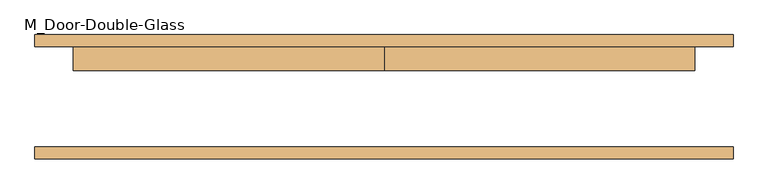
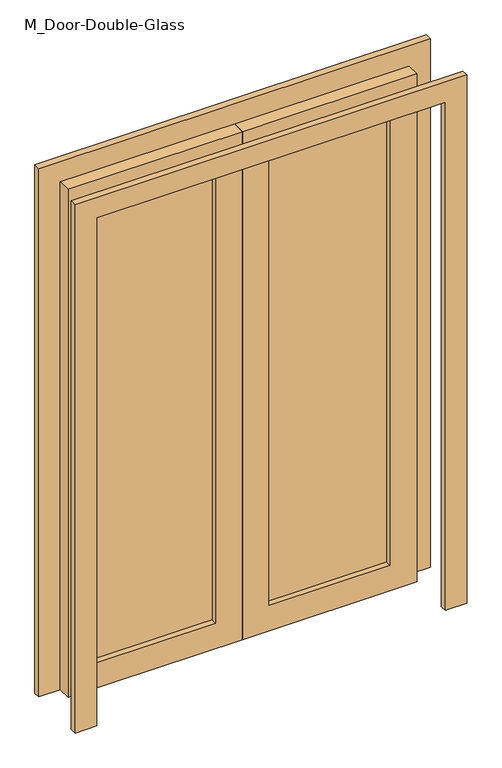
"""IFC4 building model written with IfcOpenShell, lengths in millimetres: door geometry, M_Door-Double-Glass : 130x210cm Kapı."""

import ifcopenshell
import ifcopenshell.guid

model = None  # the IFC model being written
_history = None  # IfcOwnerHistory: only IFC2X3 demands one
_inside = {}  # id of a spatial element -> (the spatial element, [elements in it])
_under = {}  # id of a project, library or spatial element -> (it, [spatial elements below it])
_declared = {}  # id of a project -> (the project, [libraries it declares])
_typed = {}  # id of a type object -> (the type object, [elements of that type])
_made_of = {}  # id of a material, layer set ... -> (it, [elements and type objects made of it])


def new_model(schema):
    """Start an empty IFC model of exactly this schema.

    Asked for "IFC4X3", IfcOpenShell would pick the latest addendum, in which some entities
    have other attributes; the version numbers below select the first issue.
    IFC2X3 requires an IfcOwnerHistory on every rooted entity: one is made here for all.
    """
    global model, _history
    if schema == "IFC4X3":
        model = ifcopenshell.file(schema_version=(4, 3, 0, 0))
    else:
        model = ifcopenshell.file(schema=schema)
    _inside.clear()
    _under.clear()
    _declared.clear()
    _typed.clear()
    _made_of.clear()
    _history = None
    if model.schema == "IFC2X3":
        org = make("IfcOrganization", Name="unknown")
        user = make(
            "IfcPersonAndOrganization",
            ThePerson=make("IfcPerson", FamilyName="unknown"),
            TheOrganization=org,
        )
        app = make(
            "IfcApplication",
            ApplicationDeveloper=org,
            Version="unknown",
            ApplicationFullName="unknown",
            ApplicationIdentifier="unknown",
        )
        _history = make(
            "IfcOwnerHistory",
            OwningUser=user,
            OwningApplication=app,
            ChangeAction="ADDED",
            CreationDate=0,
        )
    return model


def make(cls, **values):
    """One entity of the class cls with the attributes given. An attribute that is None is left unset."""
    return model.create_entity(
        cls, **{name: value for name, value in values.items() if value is not None}
    )


def rooted(cls, **values):
    """An entity with a GlobalId (a new one), such as an element, a storey or a relation."""
    return make(cls, GlobalId=ifcopenshell.guid.new(), OwnerHistory=_history, **values)


def si_unit(unit_type, name, prefix=None):
    """IfcSIUnit, for example si_unit("LENGTHUNIT", "METRE", prefix="MILLI")."""
    return make("IfcSIUnit", UnitType=unit_type, Prefix=prefix, Name=name)


def assignment(units):
    """IfcUnitAssignment: the units of a project."""
    return None if units is None else make("IfcUnitAssignment", Units=units)


def point(xyz):
    """IfcCartesianPoint."""
    return None if xyz is None else make("IfcCartesianPoint", Coordinates=xyz)


def direction(xyz):
    """IfcDirection."""
    return None if xyz is None else make("IfcDirection", DirectionRatios=xyz)


def frame(location, z_axis=None, x_axis=None):
    """IfcAxis2Placement3D, a coordinate frame: its origin and axes. An axis left out is left unset."""
    return make(
        "IfcAxis2Placement3D",
        Location=point(location),
        Axis=direction(z_axis),
        RefDirection=direction(x_axis),
    )


def origin():
    """The frame at (0, 0, 0) with its axes left unset."""
    return frame((0.0, 0.0, 0.0))


def place(relative_to, where):
    """IfcLocalPlacement: puts the frame where relative to a parent placement (None: the world)."""
    return make(
        "IfcLocalPlacement", PlacementRelTo=relative_to, RelativePlacement=where
    )


def context(
    kind, dimensions, precision=None, world=None, true_north=None, identifier=None
):
    """IfcGeometricRepresentationContext, for example the 3D "Model" context."""
    return make(
        "IfcGeometricRepresentationContext",
        ContextIdentifier=identifier,
        ContextType=kind,
        CoordinateSpaceDimension=dimensions,
        Precision=precision,
        WorldCoordinateSystem=world,
        TrueNorth=true_north,
    )


def project(units=None, contexts=None):
    """IfcProject with its units and contexts."""
    return rooted(
        "IfcProject",
        Name="project",
        RepresentationContexts=contexts,
        UnitsInContext=assignment(units),
    )


def spatial(cls, under=None, at=None, **own):
    """A site, building, storey or space (cls), placed at a placement, below another one or the project."""
    s = rooted(cls, ObjectPlacement=at, **own)
    if under is not None:
        _under.setdefault(under.id(), (under, []))[1].append(s)
    return s


def polyline(points):
    """IfcPolyline through the points."""
    return make("IfcPolyline", Points=[point(p) for p in points])


def outline(outer, holes=None, kind="AREA"):
    """IfcArbitraryClosedProfileDef: a profile drawn as a closed curve; with holes, ...WithVoids."""
    if holes is None:
        return make("IfcArbitraryClosedProfileDef", ProfileType=kind, OuterCurve=outer)
    return make(
        "IfcArbitraryProfileDefWithVoids",
        ProfileType=kind,
        OuterCurve=outer,
        InnerCurves=holes,
    )


def extrude(swept, where, along, depth):
    """IfcExtrudedAreaSolid: the profile swept, set in the frame where, extruded along a direction by depth."""
    return make(
        "IfcExtrudedAreaSolid",
        SweptArea=swept,
        Position=where,
        ExtrudedDirection=direction(along),
        Depth=depth,
    )


def shape(context_of_items, identifier, shape_type, items):
    """IfcShapeRepresentation: the items that make up one representation, for example the "Body"."""
    return make(
        "IfcShapeRepresentation",
        ContextOfItems=context_of_items,
        RepresentationIdentifier=identifier,
        RepresentationType=shape_type,
        Items=items,
    )


def source(mapping_origin, context_of_items, identifier, shape_type, items):
    """IfcRepresentationMap: a shape defined once, which mapped items show again and again."""
    return make(
        "IfcRepresentationMap",
        MappingOrigin=mapping_origin,
        MappedRepresentation=shape(context_of_items, identifier, shape_type, items),
    )


def transform(
    local_origin,
    x_axis=None,
    y_axis=None,
    z_axis=None,
    scale=None,
    scale2=None,
    scale3=None,
    uniform=True,
):
    """IfcCartesianTransformationOperator3D, or its non-uniform kind. x_axis, y_axis, z_axis: its Axis1, 2, 3."""
    if uniform:
        return make(
            "IfcCartesianTransformationOperator3D",
            Axis1=direction(x_axis),
            Axis2=direction(y_axis),
            LocalOrigin=point(local_origin),
            Scale=scale,
            Axis3=direction(z_axis),
        )
    return make(
        "IfcCartesianTransformationOperator3DnonUniform",
        Axis1=direction(x_axis),
        Axis2=direction(y_axis),
        LocalOrigin=point(local_origin),
        Scale=scale,
        Axis3=direction(z_axis),
        Scale2=scale2,
        Scale3=scale3,
    )


def mapped(mapping_source, mapping_target):
    """IfcMappedItem: shows the shape of a source again, moved by a transform."""
    return make(
        "IfcMappedItem", MappingSource=mapping_source, MappingTarget=mapping_target
    )


def made_of(thing, what):
    """Note that an element or type object is made of a material, layer set ...; save() writes the relation."""
    if what is not None:
        _made_of.setdefault(what.id(), (what, []))[1].append(thing)
    return thing


def element(
    cls,
    number,
    at=None,
    inside=None,
    cuts=None,
    type_object=None,
    material=None,
    context=None,
    identifier="Body",
    shape_type=None,
    held_by="IfcProductDefinitionShape",
    body=None,
    shapes=None,
    **own,
):
    """One element of the class cls, such as IfcWall. Its Tag is "e" and its number.

    at: its placement. inside: the storey or other place that contains it. cuts: it is an
    opening in that element (IfcRelVoidsElement). A single representation is given by context,
    identifier, shape_type and body (its items); several are given by shapes. held_by: the class
    of the entity that holds the representations. save() writes the other relations.
    """
    e = rooted(cls, Tag="e%d" % number, ObjectPlacement=at, **own)
    if body is not None:
        shapes = [shape(context, identifier, shape_type, body)]
    if shapes is not None:
        e.Representation = make(held_by, Representations=shapes)
    if inside is not None:
        _inside.setdefault(inside.id(), (inside, []))[1].append(e)
    if cuts is not None:
        rooted(
            "IfcRelVoidsElement", RelatingBuildingElement=cuts, RelatedOpeningElement=e
        )
    if type_object is not None:
        _typed.setdefault(type_object.id(), (type_object, []))[1].append(e)
    return made_of(e, material)


def aggregate(whole, parts):
    """IfcRelAggregates: a whole, such as a stair, and the parts it consists of."""
    return rooted("IfcRelAggregates", RelatingObject=whole, RelatedObjects=parts)


def save(model, path):
    """Write the relations noted so far, then the file.

    IfcRelAggregates (storeys below a building ...), IfcRelContainedInSpatialStructure (elements
    in a storey), IfcRelDefinesByType, IfcRelAssociatesMaterial and IfcRelDeclares: one each for
    every whole, place, type object, material and project.
    """
    for whole, parts in _under.values():
        aggregate(whole, parts)
    for where, things in _inside.values():
        rooted(
            "IfcRelContainedInSpatialStructure",
            RelatedElements=things,
            RelatingStructure=where,
        )
    for kind, things in _typed.values():
        rooted("IfcRelDefinesByType", RelatedObjects=things, RelatingType=kind)
    for what, things in _made_of.values():
        rooted("IfcRelAssociatesMaterial", RelatedObjects=things, RelatingMaterial=what)
    for by, libraries in _declared.values():
        rooted("IfcRelDeclares", RelatingContext=by, RelatedDefinitions=libraries)
    model.write(path)


def m_door_double_glass_87eabaac(model_context):
    return source(origin(), model_context, "Body", "SweptSolid", [
        extrude(outline(polyline([(2000.0, -650.0), (0.0, -650.0), (0.0, 0.0), (2000.0, 0.0), (2000.0, -650.0)]), holes=[polyline([(1900.0, -550.0), (1900.0, -100.0), (100.0, -100.0), (100.0, -550.0), (1900.0, -550.0)])]), frame((0.0, 57.38125, 0.0), z_axis=(0.0, 1.0, 0.0), x_axis=(0.0, 0.0, 1.0)), (0.0, 0.0, 1.0), 50.0),
        extrude(outline(polyline([(2000.0, 650.0), (2000.0, 0.0), (0.0, 0.0), (0.0, 650.0), (2000.0, 650.0)]), holes=[polyline([(1900.0, 550.0), (100.0, 550.0), (100.0, 100.0), (1900.0, 100.0), (1900.0, 550.0)])]), frame((0.0, 57.38125, 0.0), z_axis=(0.0, 1.0, 0.0), x_axis=(0.0, 0.0, 1.0)), (0.0, 0.0, 1.0), 50.0),
        extrude(outline(polyline([(100.0, 85.55625), (550.0, 85.55625), (550.0, 79.20625), (100.0, 79.20625), (100.0, 85.55625)])), frame((0.0, 0.0, 100.0), z_axis=(0.0, 0.0, 1.0), x_axis=(1.0, 0.0, 0.0)), (0.0, 0.0, 1.0), 1800.0),
        extrude(outline(polyline([(-550.0, 85.55625), (-100.0, 85.55625), (-100.0, 79.20625), (-550.0, 79.20625), (-550.0, 85.55625)])), frame((0.0, 0.0, 100.0), z_axis=(0.0, 0.0, 1.0), x_axis=(1.0, 0.0, 0.0)), (0.0, 0.0, 1.0), 1800.0),
        extrude(outline(polyline([(0.0, 730.0), (2080.0, 730.0), (2080.0, -730.0), (0.0, -730.0), (0.0, -650.0), (2000.0, -650.0), (2000.0, 650.0), (0.0, 650.0), (0.0, 730.0)])), frame((0.0, 107.38125, 0.0), z_axis=(0.0, 1.0, 0.0), x_axis=(0.0, 0.0, 1.0)), (0.0, 0.0, 1.0), 25.0),
        extrude(outline(polyline([(0.0, 730.0), (2080.0, 730.0), (2080.0, -730.0), (0.0, -730.0), (0.0, -650.0), (2000.0, -650.0), (2000.0, 650.0), (0.0, 650.0), (0.0, 730.0)])), frame((0.0, -127.61875, 0.0), z_axis=(0.0, 1.0, 0.0), x_axis=(0.0, 0.0, 1.0)), (0.0, 0.0, 1.0), 25.0),
    ])


if __name__ == "__main__":
    model = new_model("IFC4")
    model_context = context("Model", 3, world=origin())
    ifc_project = project(units=[si_unit("LENGTHUNIT", "METRE", prefix="MILLI")], contexts=[model_context])
    site = spatial("IfcSite", under=ifc_project)
    building = spatial("IfcBuilding", under=site)
    placement = place(None, origin())
    m_door_double_glass_shape = m_door_double_glass_87eabaac(model_context)
    element("IfcDoor", 1, ObjectType="M_Door-Double-Glass : 130x210cm Kapı", at=placement, inside=building, context=model_context, shape_type="MappedRepresentation", body=[
        mapped(m_door_double_glass_shape, transform((0.0, 0.0, 0.0), x_axis=(1.0, 0.0, 0.0), y_axis=(0.0, 1.0, 0.0), z_axis=(0.0, 0.0, 1.0))),
    ])
    save(model, "model.ifc")

# Revit data of these elements
# Type "M_Door-Double-Glass : 130x210cm Kapı"
#   Type Mark = "42"
#   Construction Type Id = "opn-d45"
#   Assembly Code = "C1020"
#   Analytic Construction = "Wood frame, double glass door "
#   W = 65.00 cm
#   Thickness = 5.00 cm
#   Thermal Resistance (R) = 0.31964 (m²·K)/W
#   Swing Angle [instance default] = 90.00°
#   Heat Transfer Coefficient (U) = 3.12872 W/(m²·K)
#   Height = 200.00 cm
#   Bottom Rail = 10.00 cm
#   Top Rail = 10.00 cm
#   Stiles = 10.00 cm
#   Trim Projection = 2.50 cm
#   Trim Width = 8.00 cm
#   Width = 130.00 cm
#   Define Thermal Properties by = 1
#   Glazing = Glass
#   Panel Material = Wood - Birch - Solid Stained Light Low Gloss
#   Trim Material = Paint - Sienna
#   Visual Light Transmittance = 0
#   Solar Heat Gain Coefficient = 0
#   Function = (empty or 0)
#   Wall Closure = (empty or 0)
# Element 1 (IfcDoor, "M_Door-Double-Glass : 130x210cm Kapı")
#   Materials on its faces: "Wood - Birch - Solid Stained Light Low Gloss", "Paint - Sienna", "Glass"
# Materials
#   "Glass": class "Glass", colour RGB 0 128 192, transparency 0.9, Description = "Soda Lime Glass", Cost = 0
#   "Wood - Birch - Solid Stained Light Low Gloss": class "Wood", colour RGB 210 159 95, transparency 0, Cost = 0
#   "Paint - Sienna": class "Miscellaneous", colour RGB 118 70 51, transparency 0, Cost = 0
